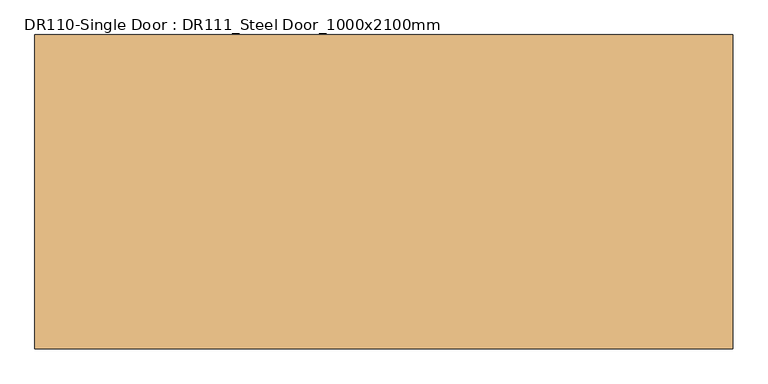
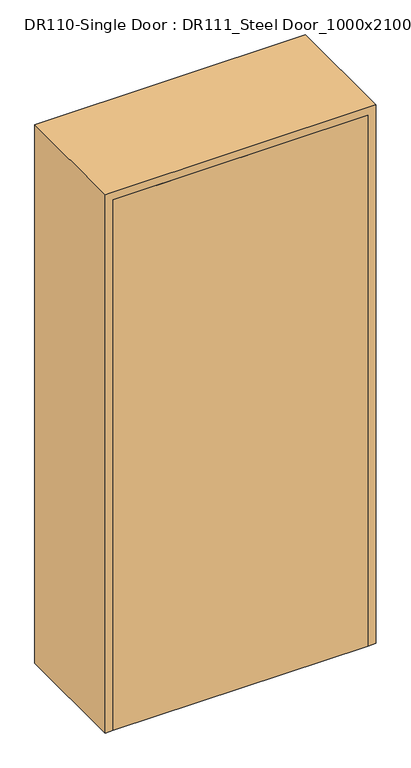
"""IFC4 building model written with IfcOpenShell, lengths in millimetres: door geometry, DR110-Single Door : DR111_Steel Door_1000x2100mm."""

import ifcopenshell
import ifcopenshell.guid

model = None  # the IFC model being written
_history = None  # IfcOwnerHistory: only IFC2X3 demands one
_inside = {}  # id of a spatial element -> (the spatial element, [elements in it])
_under = {}  # id of a project, library or spatial element -> (it, [spatial elements below it])
_declared = {}  # id of a project -> (the project, [libraries it declares])
_typed = {}  # id of a type object -> (the type object, [elements of that type])
_made_of = {}  # id of a material, layer set ... -> (it, [elements and type objects made of it])


def new_model(schema):
    """Start an empty IFC model of exactly this schema.

    Asked for "IFC4X3", IfcOpenShell would pick the latest addendum, in which some entities
    have other attributes; the version numbers below select the first issue.
    IFC2X3 requires an IfcOwnerHistory on every rooted entity: one is made here for all.
    """
    global model, _history
    if schema == "IFC4X3":
        model = ifcopenshell.file(schema_version=(4, 3, 0, 0))
    else:
        model = ifcopenshell.file(schema=schema)
    _inside.clear()
    _under.clear()
    _declared.clear()
    _typed.clear()
    _made_of.clear()
    _history = None
    if model.schema == "IFC2X3":
        org = make("IfcOrganization", Name="unknown")
        user = make(
            "IfcPersonAndOrganization",
            ThePerson=make("IfcPerson", FamilyName="unknown"),
            TheOrganization=org,
        )
        app = make(
            "IfcApplication",
            ApplicationDeveloper=org,
            Version="unknown",
            ApplicationFullName="unknown",
            ApplicationIdentifier="unknown",
        )
        _history = make(
            "IfcOwnerHistory",
            OwningUser=user,
            OwningApplication=app,
            ChangeAction="ADDED",
            CreationDate=0,
        )
    return model


def make(cls, **values):
    """One entity of the class cls with the attributes given. An attribute that is None is left unset."""
    return model.create_entity(
        cls, **{name: value for name, value in values.items() if value is not None}
    )


def rooted(cls, **values):
    """An entity with a GlobalId (a new one), such as an element, a storey or a relation."""
    return make(cls, GlobalId=ifcopenshell.guid.new(), OwnerHistory=_history, **values)


def si_unit(unit_type, name, prefix=None):
    """IfcSIUnit, for example si_unit("LENGTHUNIT", "METRE", prefix="MILLI")."""
    return make("IfcSIUnit", UnitType=unit_type, Prefix=prefix, Name=name)


def assignment(units):
    """IfcUnitAssignment: the units of a project."""
    return None if units is None else make("IfcUnitAssignment", Units=units)


def point(xyz):
    """IfcCartesianPoint."""
    return None if xyz is None else make("IfcCartesianPoint", Coordinates=xyz)


def direction(xyz):
    """IfcDirection."""
    return None if xyz is None else make("IfcDirection", DirectionRatios=xyz)


def frame(location, z_axis=None, x_axis=None):
    """IfcAxis2Placement3D, a coordinate frame: its origin and axes. An axis left out is left unset."""
    return make(
        "IfcAxis2Placement3D",
        Location=point(location),
        Axis=direction(z_axis),
        RefDirection=direction(x_axis),
    )


def origin():
    """The frame at (0, 0, 0) with its axes left unset."""
    return frame((0.0, 0.0, 0.0))


def origin_with_axes():
    """The frame at (0, 0, 0) with the z axis (0, 0, 1) and the x axis (1, 0, 0) written out."""
    return frame((0.0, 0.0, 0.0), z_axis=(0.0, 0.0, 1.0), x_axis=(1.0, 0.0, 0.0))


def place(relative_to, where):
    """IfcLocalPlacement: puts the frame where relative to a parent placement (None: the world)."""
    return make(
        "IfcLocalPlacement", PlacementRelTo=relative_to, RelativePlacement=where
    )


def context(
    kind, dimensions, precision=None, world=None, true_north=None, identifier=None
):
    """IfcGeometricRepresentationContext, for example the 3D "Model" context."""
    return make(
        "IfcGeometricRepresentationContext",
        ContextIdentifier=identifier,
        ContextType=kind,
        CoordinateSpaceDimension=dimensions,
        Precision=precision,
        WorldCoordinateSystem=world,
        TrueNorth=true_north,
    )


def project(units=None, contexts=None):
    """IfcProject with its units and contexts."""
    return rooted(
        "IfcProject",
        Name="project",
        RepresentationContexts=contexts,
        UnitsInContext=assignment(units),
    )


def spatial(cls, under=None, at=None, **own):
    """A site, building, storey or space (cls), placed at a placement, below another one or the project."""
    s = rooted(cls, ObjectPlacement=at, **own)
    if under is not None:
        _under.setdefault(under.id(), (under, []))[1].append(s)
    return s


def polyline(points):
    """IfcPolyline through the points."""
    return make("IfcPolyline", Points=[point(p) for p in points])


def outline(outer, holes=None, kind="AREA"):
    """IfcArbitraryClosedProfileDef: a profile drawn as a closed curve; with holes, ...WithVoids."""
    if holes is None:
        return make("IfcArbitraryClosedProfileDef", ProfileType=kind, OuterCurve=outer)
    return make(
        "IfcArbitraryProfileDefWithVoids",
        ProfileType=kind,
        OuterCurve=outer,
        InnerCurves=holes,
    )


def extrude(swept, where, along, depth):
    """IfcExtrudedAreaSolid: the profile swept, set in the frame where, extruded along a direction by depth."""
    return make(
        "IfcExtrudedAreaSolid",
        SweptArea=swept,
        Position=where,
        ExtrudedDirection=direction(along),
        Depth=depth,
    )


def faces_of(points, faces, orient=None, outer=None):
    """IfcFace entities. A face is a list of loops; a loop is a list of indices into points, from 0.

    orient and outer hold one flag for each loop. By default every Orientation is true, the
    first loop of a face is its IfcFaceOuterBound and the others are IfcFaceBound.
    """
    made = []
    for i, loops in enumerate(faces):
        bounds = []
        for j, loop in enumerate(loops):
            is_outer = j == 0 if outer is None else outer[i][j]
            bounds.append(
                make(
                    "IfcFaceOuterBound" if is_outer else "IfcFaceBound",
                    Bound=make("IfcPolyLoop", Polygon=[points[k] for k in loop]),
                    Orientation=True if orient is None else orient[i][j],
                )
            )
        made.append(make("IfcFace", Bounds=bounds))
    return made


def faceted_brep(points, faces, orient=None, outer=None, voids=None):
    """IfcFacetedBrep: a solid bounded by flat faces; with voids (closed shells), ...WithVoids."""
    shared = [point(p) for p in points]
    hull = make("IfcClosedShell", CfsFaces=faces_of(shared, faces, orient, outer))
    if voids is None:
        return make("IfcFacetedBrep", Outer=hull)
    return make(
        "IfcFacetedBrepWithVoids",
        Outer=hull,
        Voids=[
            make(cls, CfsFaces=faces_of(shared, fs, o, b)) for cls, fs, o, b in voids
        ],
    )


def shape(context_of_items, identifier, shape_type, items):
    """IfcShapeRepresentation: the items that make up one representation, for example the "Body"."""
    return make(
        "IfcShapeRepresentation",
        ContextOfItems=context_of_items,
        RepresentationIdentifier=identifier,
        RepresentationType=shape_type,
        Items=items,
    )


def source(mapping_origin, context_of_items, identifier, shape_type, items):
    """IfcRepresentationMap: a shape defined once, which mapped items show again and again."""
    return make(
        "IfcRepresentationMap",
        MappingOrigin=mapping_origin,
        MappedRepresentation=shape(context_of_items, identifier, shape_type, items),
    )


def transform(
    local_origin,
    x_axis=None,
    y_axis=None,
    z_axis=None,
    scale=None,
    scale2=None,
    scale3=None,
    uniform=True,
):
    """IfcCartesianTransformationOperator3D, or its non-uniform kind. x_axis, y_axis, z_axis: its Axis1, 2, 3."""
    if uniform:
        return make(
            "IfcCartesianTransformationOperator3D",
            Axis1=direction(x_axis),
            Axis2=direction(y_axis),
            LocalOrigin=point(local_origin),
            Scale=scale,
            Axis3=direction(z_axis),
        )
    return make(
        "IfcCartesianTransformationOperator3DnonUniform",
        Axis1=direction(x_axis),
        Axis2=direction(y_axis),
        LocalOrigin=point(local_origin),
        Scale=scale,
        Axis3=direction(z_axis),
        Scale2=scale2,
        Scale3=scale3,
    )


def mapped(mapping_source, mapping_target):
    """IfcMappedItem: shows the shape of a source again, moved by a transform."""
    return make(
        "IfcMappedItem", MappingSource=mapping_source, MappingTarget=mapping_target
    )


def made_of(thing, what):
    """Note that an element or type object is made of a material, layer set ...; save() writes the relation."""
    if what is not None:
        _made_of.setdefault(what.id(), (what, []))[1].append(thing)
    return thing


def element(
    cls,
    number,
    at=None,
    inside=None,
    cuts=None,
    type_object=None,
    material=None,
    context=None,
    identifier="Body",
    shape_type=None,
    held_by="IfcProductDefinitionShape",
    body=None,
    shapes=None,
    **own,
):
    """One element of the class cls, such as IfcWall. Its Tag is "e" and its number.

    at: its placement. inside: the storey or other place that contains it. cuts: it is an
    opening in that element (IfcRelVoidsElement). A single representation is given by context,
    identifier, shape_type and body (its items); several are given by shapes. held_by: the class
    of the entity that holds the representations. save() writes the other relations.
    """
    e = rooted(cls, Tag="e%d" % number, ObjectPlacement=at, **own)
    if body is not None:
        shapes = [shape(context, identifier, shape_type, body)]
    if shapes is not None:
        e.Representation = make(held_by, Representations=shapes)
    if inside is not None:
        _inside.setdefault(inside.id(), (inside, []))[1].append(e)
    if cuts is not None:
        rooted(
            "IfcRelVoidsElement", RelatingBuildingElement=cuts, RelatedOpeningElement=e
        )
    if type_object is not None:
        _typed.setdefault(type_object.id(), (type_object, []))[1].append(e)
    return made_of(e, material)


def aggregate(whole, parts):
    """IfcRelAggregates: a whole, such as a stair, and the parts it consists of."""
    return rooted("IfcRelAggregates", RelatingObject=whole, RelatedObjects=parts)


def save(model, path):
    """Write the relations noted so far, then the file.

    IfcRelAggregates (storeys below a building ...), IfcRelContainedInSpatialStructure (elements
    in a storey), IfcRelDefinesByType, IfcRelAssociatesMaterial and IfcRelDeclares: one each for
    every whole, place, type object, material and project.
    """
    for whole, parts in _under.values():
        aggregate(whole, parts)
    for where, things in _inside.values():
        rooted(
            "IfcRelContainedInSpatialStructure",
            RelatedElements=things,
            RelatingStructure=where,
        )
    for kind, things in _typed.values():
        rooted("IfcRelDefinesByType", RelatedObjects=things, RelatingType=kind)
    for what, things in _made_of.values():
        rooted("IfcRelAssociatesMaterial", RelatedObjects=things, RelatingMaterial=what)
    for by, libraries in _declared.values():
        rooted("IfcRelDeclares", RelatingContext=by, RelatedDefinitions=libraries)
    model.write(path)


def dr110_single_door_dr111_steel_door_1000x2100mm_3adf1b50(model_context):
    return source(origin(), model_context, "Body", "SolidModel", [
        extrude(outline(polyline([(470.0, -225.0), (-470.0, -225.0), (-470.0, -190.0), (470.0, -190.0), (470.0, -225.0)])), origin_with_axes(), (0.0, 0.0, 1.0), 2070.0),
        faceted_brep([(470.0, -225.0, 0.0), (470.0, -190.0, 0.0), (450.0, -190.0, 0.0), (450.0, 190.0, 0.0), (470.0, 190.0, 0.0), (470.0, 225.0, 0.0), (500.0, 225.0, 0.0), (500.0, -225.0, 0.0), (500.0, -225.0, 2100.0), (-500.0, -225.0, 2100.0), (-500.0, -225.0, 0.0), (-470.0, -225.0, 0.0), (-470.0, -225.0, 2070.0), (470.0, -225.0, 2070.0), (500.0, 225.0, 2100.0), (470.0, 225.0, 2070.0), (-470.0, 225.0, 2070.0), (-470.0, 225.0, 0.0), (-500.0, 225.0, 0.0), (-500.0, 225.0, 2100.0), (470.0, 190.0, 2070.0), (450.0, 190.0, 2050.0), (-450.0, 190.0, 2050.0), (-450.0, 190.0, 0.0), (-470.0, 190.0, 0.0), (-470.0, 190.0, 2070.0), (450.0, -190.0, 2050.0), (470.0, -190.0, 2070.0), (-470.0, -190.0, 2070.0), (-470.0, -190.0, 0.0), (-450.0, -190.0, 0.0), (-450.0, -190.0, 2050.0)], [[[0, 1, 2, 3, 4, 5, 6, 7]], [[7, 8, 9, 10, 11, 12, 13, 0]], [[6, 14, 8, 7]], [[5, 15, 16, 17, 18, 19, 14, 6]], [[4, 20, 15, 5]], [[3, 21, 22, 23, 24, 25, 20, 4]], [[2, 26, 21, 3]], [[1, 27, 28, 29, 30, 31, 26, 2]], [[0, 13, 27, 1]], [[12, 11, 29, 28]], [[11, 10, 18, 17, 24, 23, 30, 29]], [[19, 18, 10, 9]], [[25, 24, 17, 16]], [[31, 30, 23, 22]], [[14, 19, 9, 8]], [[20, 25, 16, 15]], [[26, 31, 22, 21]], [[13, 12, 28, 27]]]),
    ])


if __name__ == "__main__":
    model = new_model("IFC4")
    model_context = context("Model", 3, world=origin())
    ifc_project = project(units=[si_unit("LENGTHUNIT", "METRE", prefix="MILLI")], contexts=[model_context])
    site = spatial("IfcSite", under=ifc_project)
    building = spatial("IfcBuilding", under=site)
    placement = place(None, origin())
    dr110_single_door_dr111_steel_door_1000x2100mm_shape = dr110_single_door_dr111_steel_door_1000x2100mm_3adf1b50(model_context)
    element("IfcDoor", 1, ObjectType="DR110-Single Door : DR111_Steel Door_1000x2100mm", at=placement, inside=building, context=model_context, shape_type="MappedRepresentation", body=[
        mapped(dr110_single_door_dr111_steel_door_1000x2100mm_shape, transform((0.0, 0.0, 0.0), x_axis=(1.0, 0.0, 0.0), y_axis=(0.0, 1.0, 0.0), z_axis=(0.0, 0.0, 1.0))),
    ])
    save(model, "model.ifc")

# Revit data of these elements
# Project information
#   Building Name = "MAIN GATE SECURITY BUILDING"
#   Project Status = "Project Status"
#   Client Name = "현대엔지니어링"
#   Project Address = "서울시 종로구 율곡로 75(계동)"
#   Project Name = "Therma Visayas Energy Project"
#   Project Number = "-"
# Type "DR110-Single Door : DR111_Steel Door_1000x2100mm"
#   Type Mark = "SD"
#   Analytic Construction = "<None>"
#   프레임 투영 외부. = 25 mm
#   프레임 투영 내부. = 25 mm
#   프레임 폭 = 75 mm
#   Height = 2100 mm
#   Width = 1000 mm
#   Define Thermal Properties by = 1
#   문 패널 = A04AQ098-00002_Steel Door_non FP_single
#   문 프레임 = A04AQ098-00002_Steel Door_non FP_single
#   Function = (empty or 0)
#   Wall Closure = (empty or 0)
# Element 1 (IfcDoor, "DR110-Single Door : DR111_Steel Door_1000x2100mm")
#   Materials on its faces: "A04AQ098-00002_Steel Door_non FP_single"
# Materials
#   "A04AQ098-00002_Steel Door_non FP_single": class "금속", colour RGB 247 247 247, transparency 0, Description = "Steel Door", W00) Work Master Code = "A04AQ098-00002", W01) Work Master_Lv1 = "Finishing Work", W02) Work Master_Lv2 = "Door & Window Work", W03) Work Master_Spec.1 = "Steel Door w/ Steel Frame", W04) Work Master_Spec.2 = "Fire Protective Rating: N/A, Single Door", W05) Work Master_Spec.3 = "w/ Hardware & Accessories", Cost = 0
